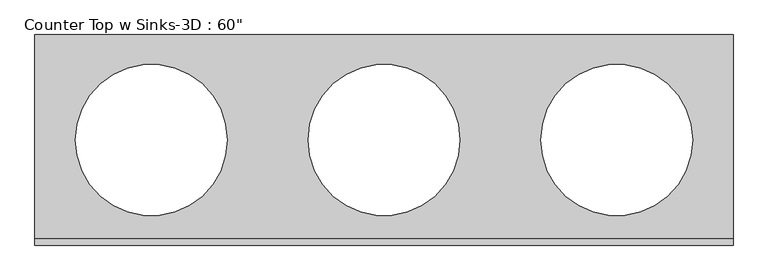
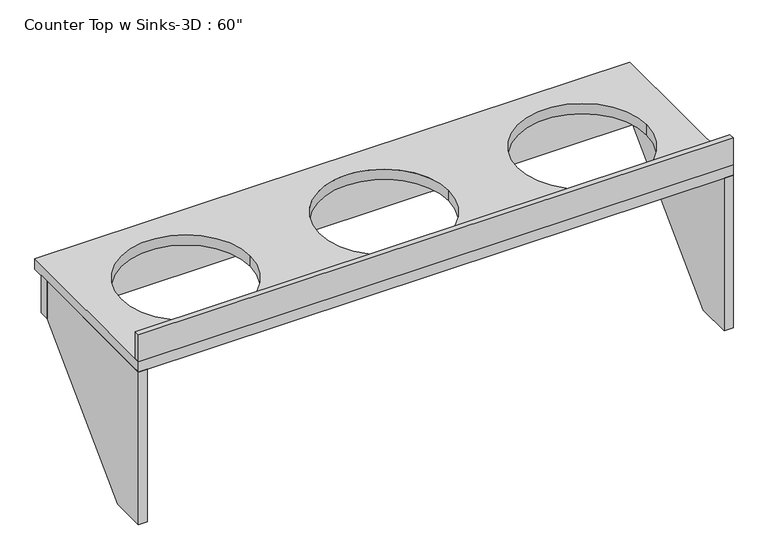
"""IFC4 building model written with IfcOpenShell, lengths in millimetres: furniture geometry."""

import ifcopenshell
import ifcopenshell.guid

model = None  # the IFC model being written
_history = None  # IfcOwnerHistory: only IFC2X3 demands one
_inside = {}  # id of a spatial element -> (the spatial element, [elements in it])
_under = {}  # id of a project, library or spatial element -> (it, [spatial elements below it])
_declared = {}  # id of a project -> (the project, [libraries it declares])
_typed = {}  # id of a type object -> (the type object, [elements of that type])
_made_of = {}  # id of a material, layer set ... -> (it, [elements and type objects made of it])


def new_model(schema):
    """Start an empty IFC model of exactly this schema.

    Asked for "IFC4X3", IfcOpenShell would pick the latest addendum, in which some entities
    have other attributes; the version numbers below select the first issue.
    IFC2X3 requires an IfcOwnerHistory on every rooted entity: one is made here for all.
    """
    global model, _history
    if schema == "IFC4X3":
        model = ifcopenshell.file(schema_version=(4, 3, 0, 0))
    else:
        model = ifcopenshell.file(schema=schema)
    _inside.clear()
    _under.clear()
    _declared.clear()
    _typed.clear()
    _made_of.clear()
    _history = None
    if model.schema == "IFC2X3":
        org = make("IfcOrganization", Name="unknown")
        user = make(
            "IfcPersonAndOrganization",
            ThePerson=make("IfcPerson", FamilyName="unknown"),
            TheOrganization=org,
        )
        app = make(
            "IfcApplication",
            ApplicationDeveloper=org,
            Version="unknown",
            ApplicationFullName="unknown",
            ApplicationIdentifier="unknown",
        )
        _history = make(
            "IfcOwnerHistory",
            OwningUser=user,
            OwningApplication=app,
            ChangeAction="ADDED",
            CreationDate=0,
        )
    return model


def make(cls, **values):
    """One entity of the class cls with the attributes given. An attribute that is None is left unset."""
    return model.create_entity(
        cls, **{name: value for name, value in values.items() if value is not None}
    )


def rooted(cls, **values):
    """An entity with a GlobalId (a new one), such as an element, a storey or a relation."""
    return make(cls, GlobalId=ifcopenshell.guid.new(), OwnerHistory=_history, **values)


def si_unit(unit_type, name, prefix=None):
    """IfcSIUnit, for example si_unit("LENGTHUNIT", "METRE", prefix="MILLI")."""
    return make("IfcSIUnit", UnitType=unit_type, Prefix=prefix, Name=name)


def assignment(units):
    """IfcUnitAssignment: the units of a project."""
    return None if units is None else make("IfcUnitAssignment", Units=units)


def point(xyz):
    """IfcCartesianPoint."""
    return None if xyz is None else make("IfcCartesianPoint", Coordinates=xyz)


def direction(xyz):
    """IfcDirection."""
    return None if xyz is None else make("IfcDirection", DirectionRatios=xyz)


def frame(location, z_axis=None, x_axis=None):
    """IfcAxis2Placement3D, a coordinate frame: its origin and axes. An axis left out is left unset."""
    return make(
        "IfcAxis2Placement3D",
        Location=point(location),
        Axis=direction(z_axis),
        RefDirection=direction(x_axis),
    )


def frame_2d(location, x_axis=None):
    """IfcAxis2Placement2D, a coordinate frame in the plane: its origin and x axis."""
    return make(
        "IfcAxis2Placement2D", Location=point(location), RefDirection=direction(x_axis)
    )


def origin():
    """The frame at (0, 0, 0) with its axes left unset."""
    return frame((0.0, 0.0, 0.0))


def place(relative_to, where):
    """IfcLocalPlacement: puts the frame where relative to a parent placement (None: the world)."""
    return make(
        "IfcLocalPlacement", PlacementRelTo=relative_to, RelativePlacement=where
    )


def context(
    kind, dimensions, precision=None, world=None, true_north=None, identifier=None
):
    """IfcGeometricRepresentationContext, for example the 3D "Model" context."""
    return make(
        "IfcGeometricRepresentationContext",
        ContextIdentifier=identifier,
        ContextType=kind,
        CoordinateSpaceDimension=dimensions,
        Precision=precision,
        WorldCoordinateSystem=world,
        TrueNorth=true_north,
    )


def project(units=None, contexts=None):
    """IfcProject with its units and contexts."""
    return rooted(
        "IfcProject",
        Name="project",
        RepresentationContexts=contexts,
        UnitsInContext=assignment(units),
    )


def spatial(cls, under=None, at=None, **own):
    """A site, building, storey or space (cls), placed at a placement, below another one or the project."""
    s = rooted(cls, ObjectPlacement=at, **own)
    if under is not None:
        _under.setdefault(under.id(), (under, []))[1].append(s)
    return s


def polyline(points):
    """IfcPolyline through the points."""
    return make("IfcPolyline", Points=[point(p) for p in points])


def circle_curve(where, radius):
    """IfcCircle in the frame where."""
    return make("IfcCircle", Position=where, Radius=radius)


def trimmed(basis, trim1, trim2, sense, master):
    """IfcTrimmedCurve: the piece of a basis curve between two trims."""
    return make(
        "IfcTrimmedCurve",
        BasisCurve=basis,
        Trim1=trim1,
        Trim2=trim2,
        SenseAgreement=sense,
        MasterRepresentation=master,
    )


def segment(curve, same_sense, transition):
    """IfcCompositeCurveSegment."""
    return make(
        "IfcCompositeCurveSegment",
        Transition=transition,
        SameSense=same_sense,
        ParentCurve=curve,
    )


def composite_curve(segments, self_intersect=None):
    """IfcCompositeCurve: segments joined end to end."""
    return make("IfcCompositeCurve", Segments=segments, SelfIntersect=self_intersect)


def outline(outer, holes=None, kind="AREA"):
    """IfcArbitraryClosedProfileDef: a profile drawn as a closed curve; with holes, ...WithVoids."""
    if holes is None:
        return make("IfcArbitraryClosedProfileDef", ProfileType=kind, OuterCurve=outer)
    return make(
        "IfcArbitraryProfileDefWithVoids",
        ProfileType=kind,
        OuterCurve=outer,
        InnerCurves=holes,
    )


def extrude(swept, where, along, depth):
    """IfcExtrudedAreaSolid: the profile swept, set in the frame where, extruded along a direction by depth."""
    return make(
        "IfcExtrudedAreaSolid",
        SweptArea=swept,
        Position=where,
        ExtrudedDirection=direction(along),
        Depth=depth,
    )


def shape(context_of_items, identifier, shape_type, items):
    """IfcShapeRepresentation: the items that make up one representation, for example the "Body"."""
    return make(
        "IfcShapeRepresentation",
        ContextOfItems=context_of_items,
        RepresentationIdentifier=identifier,
        RepresentationType=shape_type,
        Items=items,
    )


def source(mapping_origin, context_of_items, identifier, shape_type, items):
    """IfcRepresentationMap: a shape defined once, which mapped items show again and again."""
    return make(
        "IfcRepresentationMap",
        MappingOrigin=mapping_origin,
        MappedRepresentation=shape(context_of_items, identifier, shape_type, items),
    )


def transform(
    local_origin,
    x_axis=None,
    y_axis=None,
    z_axis=None,
    scale=None,
    scale2=None,
    scale3=None,
    uniform=True,
):
    """IfcCartesianTransformationOperator3D, or its non-uniform kind. x_axis, y_axis, z_axis: its Axis1, 2, 3."""
    if uniform:
        return make(
            "IfcCartesianTransformationOperator3D",
            Axis1=direction(x_axis),
            Axis2=direction(y_axis),
            LocalOrigin=point(local_origin),
            Scale=scale,
            Axis3=direction(z_axis),
        )
    return make(
        "IfcCartesianTransformationOperator3DnonUniform",
        Axis1=direction(x_axis),
        Axis2=direction(y_axis),
        LocalOrigin=point(local_origin),
        Scale=scale,
        Axis3=direction(z_axis),
        Scale2=scale2,
        Scale3=scale3,
    )


def mapped(mapping_source, mapping_target):
    """IfcMappedItem: shows the shape of a source again, moved by a transform."""
    return make(
        "IfcMappedItem", MappingSource=mapping_source, MappingTarget=mapping_target
    )


def made_of(thing, what):
    """Note that an element or type object is made of a material, layer set ...; save() writes the relation."""
    if what is not None:
        _made_of.setdefault(what.id(), (what, []))[1].append(thing)
    return thing


def element(
    cls,
    number,
    at=None,
    inside=None,
    cuts=None,
    type_object=None,
    material=None,
    context=None,
    identifier="Body",
    shape_type=None,
    held_by="IfcProductDefinitionShape",
    body=None,
    shapes=None,
    **own,
):
    """One element of the class cls, such as IfcWall. Its Tag is "e" and its number.

    at: its placement. inside: the storey or other place that contains it. cuts: it is an
    opening in that element (IfcRelVoidsElement). A single representation is given by context,
    identifier, shape_type and body (its items); several are given by shapes. held_by: the class
    of the entity that holds the representations. save() writes the other relations.
    """
    e = rooted(cls, Tag="e%d" % number, ObjectPlacement=at, **own)
    if body is not None:
        shapes = [shape(context, identifier, shape_type, body)]
    if shapes is not None:
        e.Representation = make(held_by, Representations=shapes)
    if inside is not None:
        _inside.setdefault(inside.id(), (inside, []))[1].append(e)
    if cuts is not None:
        rooted(
            "IfcRelVoidsElement", RelatingBuildingElement=cuts, RelatedOpeningElement=e
        )
    if type_object is not None:
        _typed.setdefault(type_object.id(), (type_object, []))[1].append(e)
    return made_of(e, material)


def aggregate(whole, parts):
    """IfcRelAggregates: a whole, such as a stair, and the parts it consists of."""
    return rooted("IfcRelAggregates", RelatingObject=whole, RelatedObjects=parts)


def save(model, path):
    """Write the relations noted so far, then the file.

    IfcRelAggregates (storeys below a building ...), IfcRelContainedInSpatialStructure (elements
    in a storey), IfcRelDefinesByType, IfcRelAssociatesMaterial and IfcRelDeclares: one each for
    every whole, place, type object, material and project.
    """
    for whole, parts in _under.values():
        aggregate(whole, parts)
    for where, things in _inside.values():
        rooted(
            "IfcRelContainedInSpatialStructure",
            RelatedElements=things,
            RelatingStructure=where,
        )
    for kind, things in _typed.values():
        rooted("IfcRelDefinesByType", RelatedObjects=things, RelatingType=kind)
    for what, things in _made_of.values():
        rooted("IfcRelAssociatesMaterial", RelatedObjects=things, RelatingMaterial=what)
    for by, libraries in _declared.values():
        rooted("IfcRelDeclares", RelatingContext=by, RelatedDefinitions=libraries)
    model.write(path)


def furniture_935aa8e9(model_context):
    return source(origin(), model_context, "Body", "SweptSolid", [
        extrude(outline(polyline([(198.4375, 825.5), (757.2375, 825.5), (757.2375, 685.8), (325.4375, 254.0), (198.4375, 254.0), (198.4375, 825.5)])), frame((-1116.1103038, 0.0, 0.0), z_axis=(1.0, 0.0, 0.0), x_axis=(0.0, 1.0, 0.0)), (0.0, 0.0, 1.0), 31.75),
        extrude(outline(polyline([(198.4375, 825.5), (757.2375, 825.5), (757.2375, 685.8), (325.4375, 254.0), (198.4375, 254.0), (198.4375, 825.5)])), frame((957.1646962, 0.0, 0.0), z_axis=(1.0, 0.0, 0.0), x_axis=(0.0, 1.0, 0.0)), (0.0, 0.0, 1.0), 31.75),
        extrude(outline(polyline([(-1116.1103038, 757.2375), (-1116.1103038, 795.3375), (988.9146962, 795.3375), (988.9146962, 757.2375), (-1116.1103038, 757.2375)])), frame((0.0, 0.0, 685.8), z_axis=(0.0, 0.0, 1.0), x_axis=(1.0, 0.0, 0.0)), (0.0, 0.0, 1.0), 139.7),
        extrude(outline(polyline([(988.9146962, 198.4375), (-1116.1103038, 198.4375), (-1116.1103038, 217.4875), (988.9146962, 217.4875), (988.9146962, 198.4375)])), frame((0.0, 0.0, 863.6), z_axis=(0.0, 0.0, 1.0), x_axis=(1.0, 0.0, 0.0)), (0.0, 0.0, 1.0), 101.6),
        extrude(outline(polyline([(988.9146962, 198.4375), (-1116.1103038, 198.4375), (-1116.1103038, 833.4375), (988.9146962, 833.4375), (988.9146962, 198.4375)]), holes=[composite_curve([segment(trimmed(circle_curve(frame_2d((-765.2728038, 515.9375)), 228.6), [point((-993.8728038, 515.9375))], [point((-536.6728038, 515.9375))], True, "CARTESIAN"), True, "CONTINUOUS"), segment(trimmed(circle_curve(frame_2d((-765.2728038, 515.9375)), 228.6), [point((-536.6728038, 515.9375))], [point((-993.8728038, 515.9375))], True, "CARTESIAN"), True, "CONTINUOUS")], self_intersect=False), composite_curve([segment(trimmed(circle_curve(frame_2d((638.0771962, 515.9375)), 228.6), [point((409.4771962, 515.9375))], [point((866.6771962, 515.9375))], True, "CARTESIAN"), True, "CONTINUOUS"), segment(trimmed(circle_curve(frame_2d((638.0771962, 515.9375)), 228.6), [point((866.6771962, 515.9375))], [point((409.4771962, 515.9375))], True, "CARTESIAN"), True, "CONTINUOUS")], self_intersect=False), composite_curve([segment(trimmed(circle_curve(frame_2d((-63.5978038, 515.9375)), 228.6), [point((-292.1978038, 515.9375))], [point((165.0021962, 515.9375))], True, "CARTESIAN"), True, "CONTINUOUS"), segment(trimmed(circle_curve(frame_2d((-63.5978038, 515.9375)), 228.6), [point((165.0021962, 515.9375))], [point((-292.1978038, 515.9375))], True, "CARTESIAN"), True, "CONTINUOUS")], self_intersect=False)]), frame((0.0, 0.0, 825.5), z_axis=(0.0, 0.0, 1.0), x_axis=(1.0, 0.0, 0.0)), (0.0, 0.0, 1.0), 38.1),
    ])


if __name__ == "__main__":
    model = new_model("IFC4")
    model_context = context("Model", 3, world=origin())
    ifc_project = project(units=[si_unit("LENGTHUNIT", "METRE", prefix="MILLI")], contexts=[model_context])
    site = spatial("IfcSite", under=ifc_project)
    building = spatial("IfcBuilding", under=site)
    placement = place(None, origin())
    furniture_shape = furniture_935aa8e9(model_context)
    element("IfcFurniture", 1, ObjectType="Counter Top w Sinks-3D : 60\"", at=placement, inside=building, context=model_context, shape_type="MappedRepresentation", body=[
        mapped(furniture_shape, transform((0.0, 0.0, 0.0), x_axis=(1.0, 0.0, 0.0), y_axis=(0.0, 1.0, 0.0), z_axis=(0.0, 0.0, 1.0))),
    ])
    save(model, "model.ifc")

# Revit data of these elements
# Type "Counter Top w Sinks-3D : 60\""
#   Assembly Code = "C1030400"
#   Height = 2' - 10"
#   Distance To Sink Center [instance default] = 1' - 3"
#   Clear Space = 2' - 3"
#   Counter Thickness = 0' - 1 1/2"
#   Depth = 2' - 1"
#   Length [instance default] = 5' - 0"
#   Number Of Sinks [instance default] = 2
#   Counter Top Material = Counter Top
#   Base Material = Laminate
#   Default Elevation = 0
# Element 1 (IfcFurniture, "Counter Top w Sinks-3D : 60\"")
#   Distance To Sink Center = 1' - 1 13/16"
#   Length = 6' - 10 7/8"
#   Number Of Sinks = 3
#   Materials on its faces: "Counter Top", "Laminate"
# Materials
#   "Counter Top": class "Unassigned", colour RGB 247 247 239, transparency 0
#   "Laminate": class "Unassigned", colour RGB 247 235 201, transparency 0
